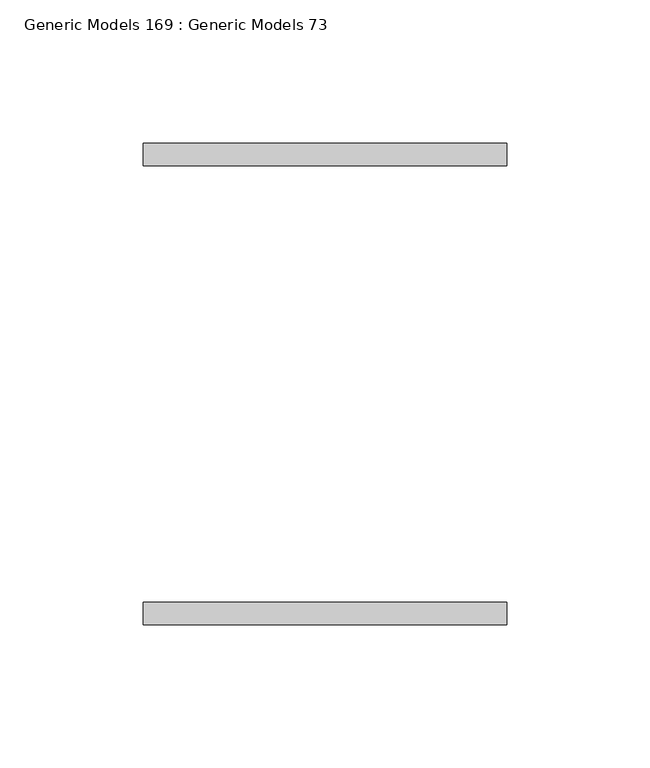
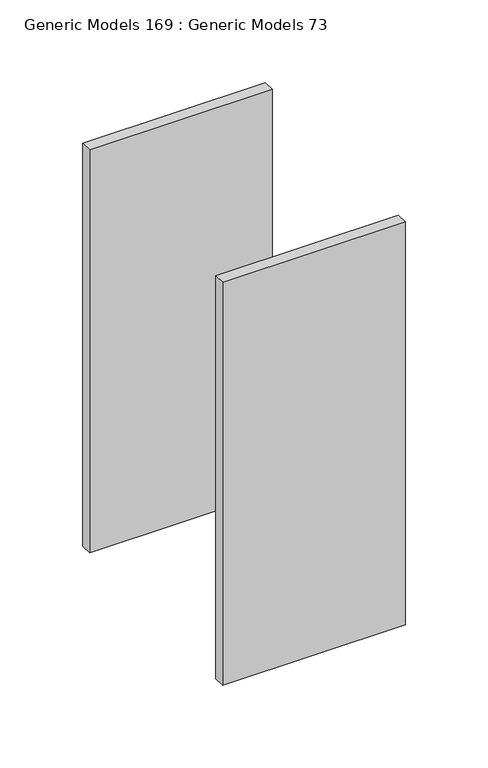
"""IFC4 building model written with IfcOpenShell, lengths in millimetres: proxy geometry, Generic Models 169 : Generic Models 73."""

from ifc_helpers import new_model, si_unit, frame, origin, place, context, project, spatial, polyline, outline, extrude, source, transform, mapped, element, save


def generic_models_169_generic_models_73_d0de1128(model_context):
    return source(origin(), model_context, "Body", "SweptSolid", [
        extrude(outline(polyline([(32053.2090778, 36491.5582942), (32053.2090778, 36483.6207942), (31926.2090778, 36483.6207942), (31926.2090778, 36491.5582942), (32053.2090778, 36491.5582942)])), frame((0.0, 0.0, 268452.944013), z_axis=(0.0, 0.0, 1.0), x_axis=(1.0, 0.0, 0.0)), (0.0, 0.0, 1.0), 296.518487),
        extrude(outline(polyline([(32053.2090778, 36331.2207942), (32053.2090778, 36323.2832942), (31926.2090778, 36323.2832942), (31926.2090778, 36331.2207942), (32053.2090778, 36331.2207942)])), frame((0.0, 0.0, 268452.944013), z_axis=(0.0, 0.0, 1.0), x_axis=(1.0, 0.0, 0.0)), (0.0, 0.0, 1.0), 296.518487),
    ])


if __name__ == "__main__":
    model = new_model("IFC4")
    model_context = context("Model", 3, world=origin())
    ifc_project = project(units=[si_unit("LENGTHUNIT", "METRE", prefix="MILLI")], contexts=[model_context])
    site = spatial("IfcSite", under=ifc_project)
    building = spatial("IfcBuilding", under=site)
    placement = place(None, origin())
    generic_models_169_generic_models_73_shape = generic_models_169_generic_models_73_d0de1128(model_context)
    element("IfcBuildingElementProxy", 1, Name="Generic Models 169 : Generic Models 73", ObjectType="Generic Models 169 : Generic Models 73", at=placement, inside=building, context=model_context, shape_type="MappedRepresentation", body=[
        mapped(generic_models_169_generic_models_73_shape, transform((0.0, 0.0, 0.0), x_axis=(1.0, 0.0, 0.0), y_axis=(0.0, 1.0, 0.0), z_axis=(0.0, 0.0, 1.0))),
    ])
    save(model, "model.ifc")

# Revit data of these elements
# Element 1 (IfcBuildingElementProxy, "Generic Models 169 : Generic Models 73")
#   Materials on its faces: "5/16 THICK GALV. SADDLE"
# Materials
#   "5/16 THICK GALV. SADDLE": class "Metal", colour RGB 199 199 199, transparency 0, Description = "Carbon steel", Cost = 0
